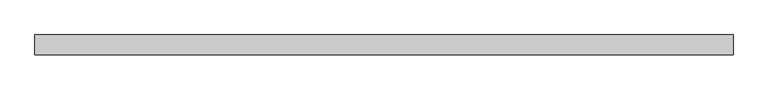
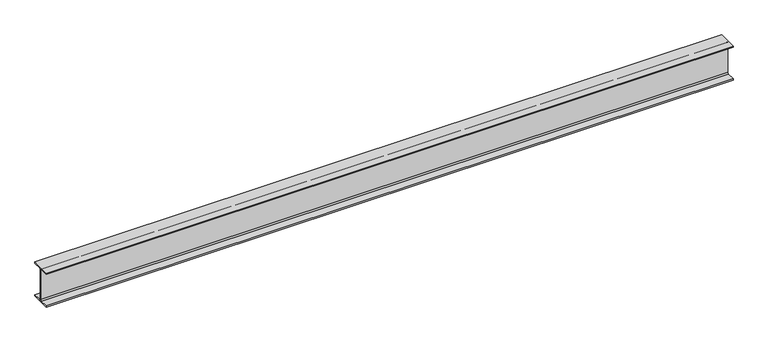
"""IFC4 building model written with IfcOpenShell, lengths in millimetres: beam geometry, Old_Steel Beam_H-KSD3502 : H_SB_ASB_H-350×175x7x11."""

import ifcopenshell
import ifcopenshell.guid

model = None  # the IFC model being written
_history = None  # IfcOwnerHistory: only IFC2X3 demands one
_inside = {}  # id of a spatial element -> (the spatial element, [elements in it])
_under = {}  # id of a project, library or spatial element -> (it, [spatial elements below it])
_declared = {}  # id of a project -> (the project, [libraries it declares])
_typed = {}  # id of a type object -> (the type object, [elements of that type])
_made_of = {}  # id of a material, layer set ... -> (it, [elements and type objects made of it])


def new_model(schema):
    """Start an empty IFC model of exactly this schema.

    Asked for "IFC4X3", IfcOpenShell would pick the latest addendum, in which some entities
    have other attributes; the version numbers below select the first issue.
    IFC2X3 requires an IfcOwnerHistory on every rooted entity: one is made here for all.
    """
    global model, _history
    if schema == "IFC4X3":
        model = ifcopenshell.file(schema_version=(4, 3, 0, 0))
    else:
        model = ifcopenshell.file(schema=schema)
    _inside.clear()
    _under.clear()
    _declared.clear()
    _typed.clear()
    _made_of.clear()
    _history = None
    if model.schema == "IFC2X3":
        org = make("IfcOrganization", Name="unknown")
        user = make(
            "IfcPersonAndOrganization",
            ThePerson=make("IfcPerson", FamilyName="unknown"),
            TheOrganization=org,
        )
        app = make(
            "IfcApplication",
            ApplicationDeveloper=org,
            Version="unknown",
            ApplicationFullName="unknown",
            ApplicationIdentifier="unknown",
        )
        _history = make(
            "IfcOwnerHistory",
            OwningUser=user,
            OwningApplication=app,
            ChangeAction="ADDED",
            CreationDate=0,
        )
    return model


def make(cls, **values):
    """One entity of the class cls with the attributes given. An attribute that is None is left unset."""
    return model.create_entity(
        cls, **{name: value for name, value in values.items() if value is not None}
    )


def rooted(cls, **values):
    """An entity with a GlobalId (a new one), such as an element, a storey or a relation."""
    return make(cls, GlobalId=ifcopenshell.guid.new(), OwnerHistory=_history, **values)


def si_unit(unit_type, name, prefix=None):
    """IfcSIUnit, for example si_unit("LENGTHUNIT", "METRE", prefix="MILLI")."""
    return make("IfcSIUnit", UnitType=unit_type, Prefix=prefix, Name=name)


def assignment(units):
    """IfcUnitAssignment: the units of a project."""
    return None if units is None else make("IfcUnitAssignment", Units=units)


def point(xyz):
    """IfcCartesianPoint."""
    return None if xyz is None else make("IfcCartesianPoint", Coordinates=xyz)


def direction(xyz):
    """IfcDirection."""
    return None if xyz is None else make("IfcDirection", DirectionRatios=xyz)


def frame(location, z_axis=None, x_axis=None):
    """IfcAxis2Placement3D, a coordinate frame: its origin and axes. An axis left out is left unset."""
    return make(
        "IfcAxis2Placement3D",
        Location=point(location),
        Axis=direction(z_axis),
        RefDirection=direction(x_axis),
    )


def frame_2d(location, x_axis=None):
    """IfcAxis2Placement2D, a coordinate frame in the plane: its origin and x axis."""
    return make(
        "IfcAxis2Placement2D", Location=point(location), RefDirection=direction(x_axis)
    )


def origin():
    """The frame at (0, 0, 0) with its axes left unset."""
    return frame((0.0, 0.0, 0.0))


def place(relative_to, where):
    """IfcLocalPlacement: puts the frame where relative to a parent placement (None: the world)."""
    return make(
        "IfcLocalPlacement", PlacementRelTo=relative_to, RelativePlacement=where
    )


def context(
    kind, dimensions, precision=None, world=None, true_north=None, identifier=None
):
    """IfcGeometricRepresentationContext, for example the 3D "Model" context."""
    return make(
        "IfcGeometricRepresentationContext",
        ContextIdentifier=identifier,
        ContextType=kind,
        CoordinateSpaceDimension=dimensions,
        Precision=precision,
        WorldCoordinateSystem=world,
        TrueNorth=true_north,
    )


def project(units=None, contexts=None):
    """IfcProject with its units and contexts."""
    return rooted(
        "IfcProject",
        Name="project",
        RepresentationContexts=contexts,
        UnitsInContext=assignment(units),
    )


def spatial(cls, under=None, at=None, **own):
    """A site, building, storey or space (cls), placed at a placement, below another one or the project."""
    s = rooted(cls, ObjectPlacement=at, **own)
    if under is not None:
        _under.setdefault(under.id(), (under, []))[1].append(s)
    return s


def polyline(points):
    """IfcPolyline through the points."""
    return make("IfcPolyline", Points=[point(p) for p in points])


def circle_curve(where, radius):
    """IfcCircle in the frame where."""
    return make("IfcCircle", Position=where, Radius=radius)


def trimmed(basis, trim1, trim2, sense, master):
    """IfcTrimmedCurve: the piece of a basis curve between two trims."""
    return make(
        "IfcTrimmedCurve",
        BasisCurve=basis,
        Trim1=trim1,
        Trim2=trim2,
        SenseAgreement=sense,
        MasterRepresentation=master,
    )


def segment(curve, same_sense, transition):
    """IfcCompositeCurveSegment."""
    return make(
        "IfcCompositeCurveSegment",
        Transition=transition,
        SameSense=same_sense,
        ParentCurve=curve,
    )


def composite_curve(segments, self_intersect=None):
    """IfcCompositeCurve: segments joined end to end."""
    return make("IfcCompositeCurve", Segments=segments, SelfIntersect=self_intersect)


def outline(outer, holes=None, kind="AREA"):
    """IfcArbitraryClosedProfileDef: a profile drawn as a closed curve; with holes, ...WithVoids."""
    if holes is None:
        return make("IfcArbitraryClosedProfileDef", ProfileType=kind, OuterCurve=outer)
    return make(
        "IfcArbitraryProfileDefWithVoids",
        ProfileType=kind,
        OuterCurve=outer,
        InnerCurves=holes,
    )


def extrude(swept, where, along, depth):
    """IfcExtrudedAreaSolid: the profile swept, set in the frame where, extruded along a direction by depth."""
    return make(
        "IfcExtrudedAreaSolid",
        SweptArea=swept,
        Position=where,
        ExtrudedDirection=direction(along),
        Depth=depth,
    )


def shape(context_of_items, identifier, shape_type, items):
    """IfcShapeRepresentation: the items that make up one representation, for example the "Body"."""
    return make(
        "IfcShapeRepresentation",
        ContextOfItems=context_of_items,
        RepresentationIdentifier=identifier,
        RepresentationType=shape_type,
        Items=items,
    )


def source(mapping_origin, context_of_items, identifier, shape_type, items):
    """IfcRepresentationMap: a shape defined once, which mapped items show again and again."""
    return make(
        "IfcRepresentationMap",
        MappingOrigin=mapping_origin,
        MappedRepresentation=shape(context_of_items, identifier, shape_type, items),
    )


def transform(
    local_origin,
    x_axis=None,
    y_axis=None,
    z_axis=None,
    scale=None,
    scale2=None,
    scale3=None,
    uniform=True,
):
    """IfcCartesianTransformationOperator3D, or its non-uniform kind. x_axis, y_axis, z_axis: its Axis1, 2, 3."""
    if uniform:
        return make(
            "IfcCartesianTransformationOperator3D",
            Axis1=direction(x_axis),
            Axis2=direction(y_axis),
            LocalOrigin=point(local_origin),
            Scale=scale,
            Axis3=direction(z_axis),
        )
    return make(
        "IfcCartesianTransformationOperator3DnonUniform",
        Axis1=direction(x_axis),
        Axis2=direction(y_axis),
        LocalOrigin=point(local_origin),
        Scale=scale,
        Axis3=direction(z_axis),
        Scale2=scale2,
        Scale3=scale3,
    )


def mapped(mapping_source, mapping_target):
    """IfcMappedItem: shows the shape of a source again, moved by a transform."""
    return make(
        "IfcMappedItem", MappingSource=mapping_source, MappingTarget=mapping_target
    )


def made_of(thing, what):
    """Note that an element or type object is made of a material, layer set ...; save() writes the relation."""
    if what is not None:
        _made_of.setdefault(what.id(), (what, []))[1].append(thing)
    return thing


def element(
    cls,
    number,
    at=None,
    inside=None,
    cuts=None,
    type_object=None,
    material=None,
    context=None,
    identifier="Body",
    shape_type=None,
    held_by="IfcProductDefinitionShape",
    body=None,
    shapes=None,
    **own,
):
    """One element of the class cls, such as IfcWall. Its Tag is "e" and its number.

    at: its placement. inside: the storey or other place that contains it. cuts: it is an
    opening in that element (IfcRelVoidsElement). A single representation is given by context,
    identifier, shape_type and body (its items); several are given by shapes. held_by: the class
    of the entity that holds the representations. save() writes the other relations.
    """
    e = rooted(cls, Tag="e%d" % number, ObjectPlacement=at, **own)
    if body is not None:
        shapes = [shape(context, identifier, shape_type, body)]
    if shapes is not None:
        e.Representation = make(held_by, Representations=shapes)
    if inside is not None:
        _inside.setdefault(inside.id(), (inside, []))[1].append(e)
    if cuts is not None:
        rooted(
            "IfcRelVoidsElement", RelatingBuildingElement=cuts, RelatedOpeningElement=e
        )
    if type_object is not None:
        _typed.setdefault(type_object.id(), (type_object, []))[1].append(e)
    return made_of(e, material)


def aggregate(whole, parts):
    """IfcRelAggregates: a whole, such as a stair, and the parts it consists of."""
    return rooted("IfcRelAggregates", RelatingObject=whole, RelatedObjects=parts)


def save(model, path):
    """Write the relations noted so far, then the file.

    IfcRelAggregates (storeys below a building ...), IfcRelContainedInSpatialStructure (elements
    in a storey), IfcRelDefinesByType, IfcRelAssociatesMaterial and IfcRelDeclares: one each for
    every whole, place, type object, material and project.
    """
    for whole, parts in _under.values():
        aggregate(whole, parts)
    for where, things in _inside.values():
        rooted(
            "IfcRelContainedInSpatialStructure",
            RelatedElements=things,
            RelatingStructure=where,
        )
    for kind, things in _typed.values():
        rooted("IfcRelDefinesByType", RelatedObjects=things, RelatingType=kind)
    for what, things in _made_of.values():
        rooted("IfcRelAssociatesMaterial", RelatedObjects=things, RelatingMaterial=what)
    for by, libraries in _declared.values():
        rooted("IfcRelDeclares", RelatingContext=by, RelatedDefinitions=libraries)
    model.write(path)


def beam_62b6306e(model_context):
    return source(origin(), model_context, "Body", "SweptSolid", [
        extrude(outline(composite_curve([segment(polyline([(82.5, -141.5), (82.5, -151.7), (-82.5, -151.7), (-82.5, -141.5), (-11.9, -141.5)]), True, "CONTINUOUS"), segment(trimmed(circle_curve(frame_2d((-11.9, -132.6)), 8.9), [point((-11.9, -141.5))], [point((-3.0, -132.6))], True, "CARTESIAN"), True, "CONTINUOUS"), segment(polyline([(-3.0, -132.6), (-3.0, 132.6)]), True, "CONTINUOUS"), segment(trimmed(circle_curve(frame_2d((-11.9, 132.6)), 8.9), [point((-3.0, 132.6))], [point((-11.9, 141.5))], True, "CARTESIAN"), True, "CONTINUOUS"), segment(polyline([(-11.9, 141.5), (-82.5, 141.5), (-82.5, 151.7), (82.5, 151.7), (82.5, 141.5), (11.9, 141.5)]), True, "CONTINUOUS"), segment(trimmed(circle_curve(frame_2d((11.9, 132.6)), 8.9), [point((11.9, 141.5))], [point((3.0, 132.6))], True, "CARTESIAN"), True, "CONTINUOUS"), segment(polyline([(3.0, 132.6), (3.0, -132.6)]), True, "CONTINUOUS"), segment(trimmed(circle_curve(frame_2d((11.9, -132.6)), 8.9), [point((3.0, -132.6))], [point((11.9, -141.5))], True, "CARTESIAN"), True, "CONTINUOUS"), segment(polyline([(11.9, -141.5), (82.5, -141.5)]), True, "CONTINUOUS")], self_intersect=False)), frame((-2889.9826898, 0.0, 0.0), z_axis=(1.0, 0.0, 0.0), x_axis=(0.0, 1.0, 0.0)), (0.0, 0.0, 1.0), 5810.1548079),
    ])


if __name__ == "__main__":
    model = new_model("IFC4")
    model_context = context("Model", 3, world=origin())
    ifc_project = project(units=[si_unit("LENGTHUNIT", "METRE", prefix="MILLI")], contexts=[model_context])
    site = spatial("IfcSite", under=ifc_project)
    building = spatial("IfcBuilding", under=site)
    placement = place(None, origin())
    beam_shape = beam_62b6306e(model_context)
    element("IfcBeam", 1, ObjectType="Old_Steel Beam_H-KSD3502 : H_SB_ASB_H-350×175x7x11", at=placement, inside=building, context=model_context, shape_type="MappedRepresentation", body=[
        mapped(beam_shape, transform((0.0, 0.0, 0.0), x_axis=(1.0, 0.0, 0.0), y_axis=(0.0, 1.0, 0.0), z_axis=(0.0, 0.0, 1.0))),
    ])
    save(model, "model.ifc")

# Revit data of these elements
# Type "Old_Steel Beam_H-KSD3502 : H_SB_ASB_H-350×175x7x11"
#   Width = 17.5 cm
#   Web Thickness = 0.7 cm
#   Web Fillet = 1.4 cm
#   Warping Constant = 282290.0 cm⁶
#   Torsional Moment of Inertia = 19.4042 cm⁴
#   Torsional Modulus = 1.0 cm³
#   Section Area = 63.14 cm²
#   Plastic Modulus weak axis = 174.0 cm³
#   Plastic Modulus strong axis = 868.0 cm³
#   Perimeter = 1.36 m²/m
#   Nominal Weight = 49.60 kgf/m
#   Moment of Inertia weak axis = 984.00 cm⁴
#   Moment of Inertia strong axis = 13600.00 cm⁴
#   Height = 35.0 cm
#   Flange Thickness = 1.1 cm
#   Elastic Modulus weak axis = 112.0 cm³
#   Elastic Modulus strong axis = 775.0 cm³
#   Centroid Vertical = 17.5 cm
#   Centroid Horizontal = 8.75 cm
#   Length [instance default] = 1.5240 m
#   Structural Material [instance default] = Steel, 45-345
#   Assembly Code = ""
# Element 1 (IfcBeam, "Old_Steel Beam_H-KSD3502 : H_SB_ASB_H-350×175x7x11")
#   Structural Material = none
# Materials
#   "Steel, 45-345": class "Metal", colour RGB 189 187 185, transparency 0, Description = "Steel 345 MPa", Cost = 0
